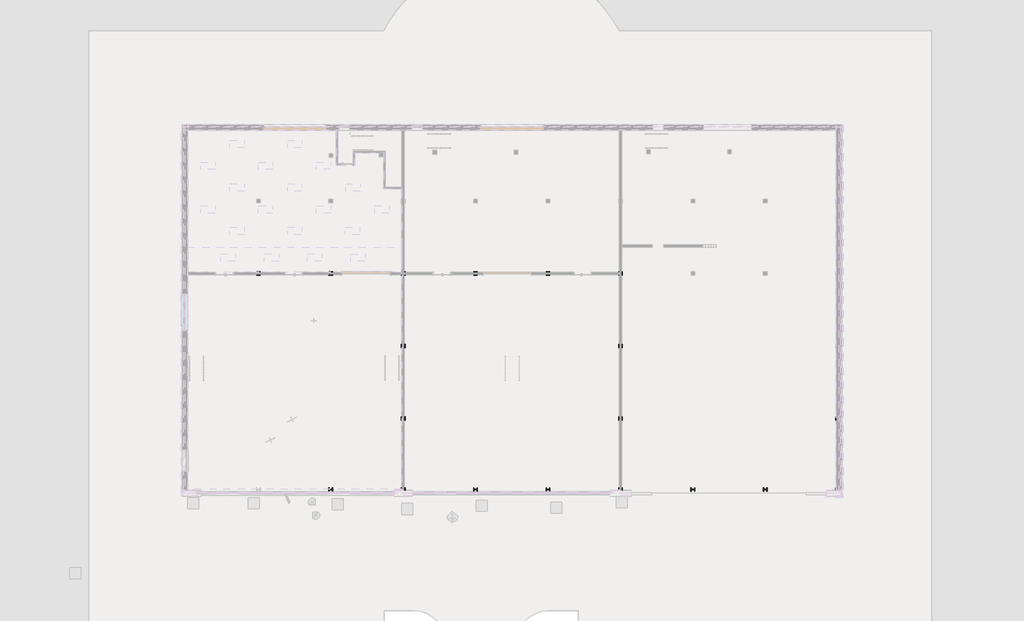
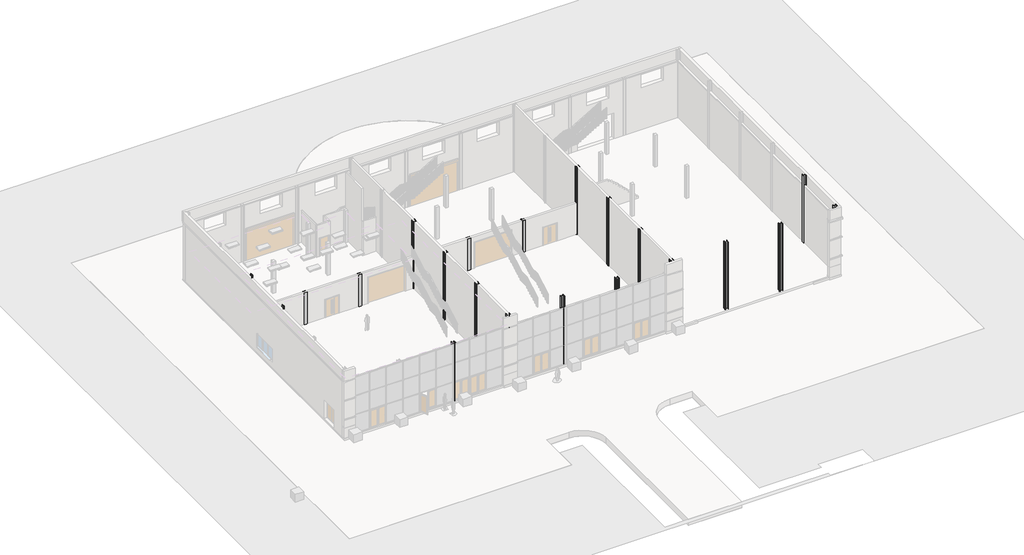
# One storey, part 5 of 13: 21 columns, 21 slabs, 8 footings.
# Revit data of these elements (continued)
# Elements 1, 2, 3, 4 (IfcColumn, "Concrete Square : 300 x 300mm")
#   Comments = ""
#   Phase Created = New Construction
#   Materials on its faces: "Concrete - Cast-in-Place Concrete"
# Elements 5, 6, 7, 8, 9, 10, 11, 12, 13, 14, 15, 16, 17, 18, 19, 20, 21 (IfcColumn, "UC-Universal Column-Column : 305x305x97UC")
#   Comments = ""
#   Structural Material = Steel, 45-345
#   Phase Created = New Construction
#   Materials on its faces: "Steel, 45-345"
# Elements 22, 23, 24, 25, 26, 27 (IfcFooting, "Wall Foundation - Commercial 1300 x 450")
#   Phase Created = New Construction
#   Materials on its faces: "Concrete, Cast In Situ"
# Elements 28, 29 (IfcFooting, "Wall Foundation - Commercial 1300 x 450")
#   Comments = ""
#   Phase Created = New Construction
#   Materials on its faces: "Concrete, Cast In Situ"
# Elements 30, 31, 32, 33, 34, 35, 36, 37, 38, 39, 40, 41, 42, 43, 44, 45, 46, 47, 48, 49, 50 (IfcSlab, "Pad Foundation-Rectangular : 1000x1000x500")
#   Comments = ""
#   Reinforcement Specs = ""
#   Mesh = ""
#   Concrete Grade = ""
#   Structural Material = Concrete - Cast-in-Place Concrete
#   Phase Created = New Construction
#   Materials on its faces: "Concrete - Cast-in-Place Concrete"
# Materials
#   "Concrete - Cast-in-Place Concrete": class "Concrete", colour RGB 192 192 192, transparency 0
#   "Steel, 45-345": class "Metal", colour RGB 247 247 247, transparency 0, Description = "Steel 345 MPa", Cost = 0
#   "Concrete, Cast In Situ": class "Concrete", colour RGB 192 192 192, transparency 0, Description = "physical material", Cost = 0
# Room at (2534.039, 34.316) mm, phase "New Construction", upper level "L0 - Ground Floor (Shadows On)", upper offset 4000 mm, lower offset 0 mm
#   Number = "1"
#   Name = "Room"
# Room at (2390.683, -14731.423) mm, phase "New Construction", upper level "L0 - Ground Floor (Shadows On)", upper offset 4000 mm, lower offset 0 mm
#   Number = "2"
#   Name = "Room"
